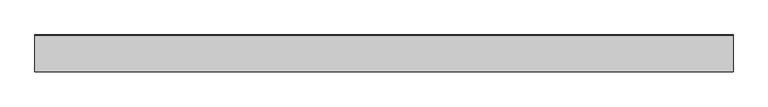
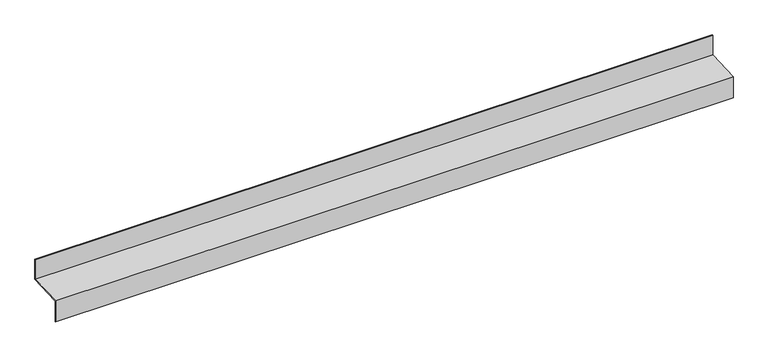
"""IFC4 building model written with IfcOpenShell, lengths in millimetres: proxy geometry, Generic Models 7:Generic Models 1:5:Generic Models 1:5 : Generic Models 7:Generic Models 1:337419:10 : Generic Models 7:Generic Models 1:5:Generic Models 1:5 : Generic Models 7:Generic Models 1:337419:311462."""

from ifc_helpers import new_model, si_unit, frame, origin, place, context, project, spatial, polyline, outline, extrude, source, transform, mapped, element, save


def generic_models_708b70e2(model_context):
    return source(origin(), model_context, "Body", "SweptSolid", [
        extrude(outline(polyline([(-579143.6477614, -76.436279), (-579145.2352614, -76.436279), (-579145.2352614, 4.0632001), (-579017.3601341, 9.3913304), (-579017.3601341, 84.3642418), (-579015.7726341, 84.3642418), (-579015.7726341, 7.8685988), (-579143.6477614, 2.5404685), (-579143.6477614, -76.436279)])), frame((593738.0867239, 0.0, 0.0), z_axis=(1.0, 0.0, 0.0), x_axis=(0.0, 1.0, 0.0)), (0.0, 0.0, 1.0), 2444.75),
    ])


if __name__ == "__main__":
    model = new_model("IFC4")
    model_context = context("Model", 3, world=origin())
    ifc_project = project(units=[si_unit("LENGTHUNIT", "METRE", prefix="MILLI")], contexts=[model_context])
    site = spatial("IfcSite", under=ifc_project)
    building = spatial("IfcBuilding", under=site)
    placement = place(None, origin())
    generic_models_shape = generic_models_708b70e2(model_context)
    element("IfcBuildingElementProxy", 1, Name="Generic Models 7:Generic Models 1:5:Generic Models 1:5 : Generic Models 7:Generic Models 1:337419:10 : Generic Models 7:Generic Models 1:5:Generic Models 1:5 : Generic Models 7:Generic Models 1:337419:311462", ObjectType="Generic Models 7:Generic Models 1:5:Generic Models 1:5 : Generic Models 7:Generic Models 1:337419:10 : Generic Models 7:Generic Models 1:5:Generic Models 1:5 : Generic Models 7:Generic Models 1:337419:311462", at=placement, inside=building, context=model_context, shape_type="MappedRepresentation", body=[
        mapped(generic_models_shape, transform((0.0, 0.0, 0.0), x_axis=(1.0, 0.0, 0.0), y_axis=(0.0, 1.0, 0.0), z_axis=(0.0, 0.0, 1.0))),
    ])
    save(model, "model.ifc")

# Revit data of these elements
# Type "Generic Models 7:Generic Models 1:5:Generic Models 1:5 : Generic Models 7:Generic Models 1:337419:10 : Generic Models 7:Generic Models 1:5:Generic Models 1:5 : Generic Models 7:Generic Models 1:337419:311462"
#   NameOverride = "Generic Models 7:Generic Models 1:5:Generic Models 1:5 : Generic Models 7:Generic Models 1:337419:311462"
#   ObjectTypeOverride = "Generic Models 1:5 : Generic Models 7:Generic Models 1:337419"
#   Reference = "Generic Models 1"
#   Tag = "311462"
# Element 1 (IfcBuildingElementProxy, "Generic Models 7:Generic Models 1:5:Generic Models 1:5 : Generic Models 7:Generic Models 1:337419:10 : Generic Models 7:Generic Models 1:5:Generic Models 1:5 : Generic Models 7:Generic Models 1:337419:311462")
#   Materials on its faces: "16 GA. STAINLESS STEEL BRAKE METAL"
# Materials
#   "16 GA. STAINLESS STEEL BRAKE METAL": class "Unassigned", colour RGB 210 209 208, transparency 0, Cost = 0
